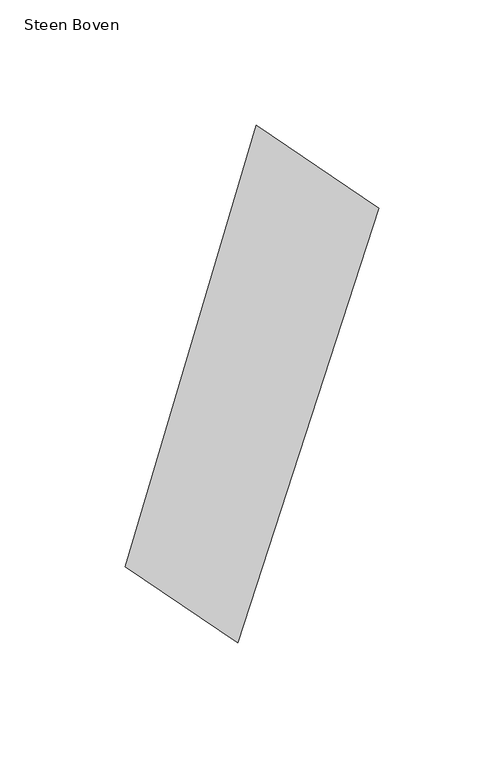
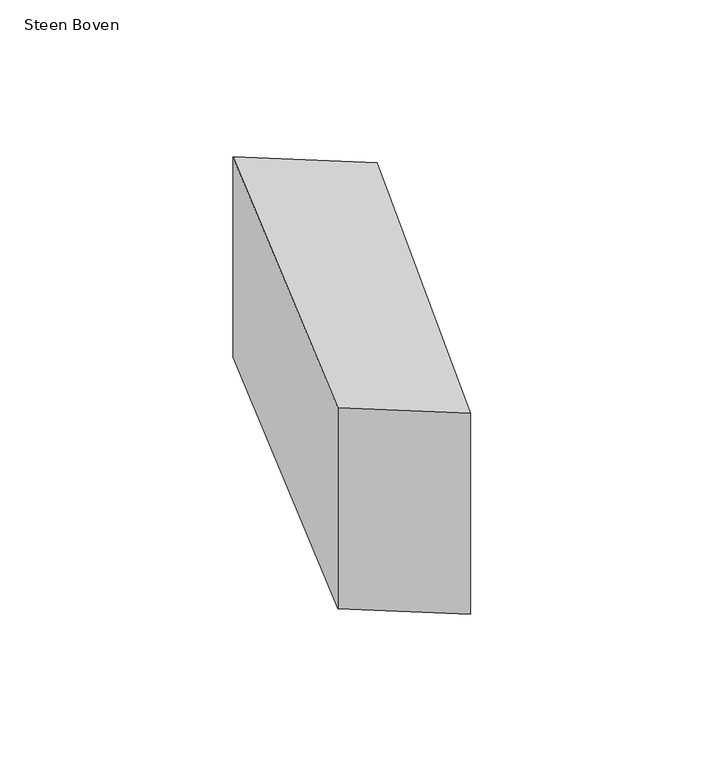
"""IFC4 building model written with IfcOpenShell, lengths in millimetres: proxy geometry, 00_GMA_steen_versie_4 : Steen Boven."""

import ifcopenshell
import ifcopenshell.guid

model = None  # the IFC model being written
_history = None  # IfcOwnerHistory: only IFC2X3 demands one
_inside = {}  # id of a spatial element -> (the spatial element, [elements in it])
_under = {}  # id of a project, library or spatial element -> (it, [spatial elements below it])
_declared = {}  # id of a project -> (the project, [libraries it declares])
_typed = {}  # id of a type object -> (the type object, [elements of that type])
_made_of = {}  # id of a material, layer set ... -> (it, [elements and type objects made of it])


def new_model(schema):
    """Start an empty IFC model of exactly this schema.

    Asked for "IFC4X3", IfcOpenShell would pick the latest addendum, in which some entities
    have other attributes; the version numbers below select the first issue.
    IFC2X3 requires an IfcOwnerHistory on every rooted entity: one is made here for all.
    """
    global model, _history
    if schema == "IFC4X3":
        model = ifcopenshell.file(schema_version=(4, 3, 0, 0))
    else:
        model = ifcopenshell.file(schema=schema)
    _inside.clear()
    _under.clear()
    _declared.clear()
    _typed.clear()
    _made_of.clear()
    _history = None
    if model.schema == "IFC2X3":
        org = make("IfcOrganization", Name="unknown")
        user = make(
            "IfcPersonAndOrganization",
            ThePerson=make("IfcPerson", FamilyName="unknown"),
            TheOrganization=org,
        )
        app = make(
            "IfcApplication",
            ApplicationDeveloper=org,
            Version="unknown",
            ApplicationFullName="unknown",
            ApplicationIdentifier="unknown",
        )
        _history = make(
            "IfcOwnerHistory",
            OwningUser=user,
            OwningApplication=app,
            ChangeAction="ADDED",
            CreationDate=0,
        )
    return model


def make(cls, **values):
    """One entity of the class cls with the attributes given. An attribute that is None is left unset."""
    return model.create_entity(
        cls, **{name: value for name, value in values.items() if value is not None}
    )


def rooted(cls, **values):
    """An entity with a GlobalId (a new one), such as an element, a storey or a relation."""
    return make(cls, GlobalId=ifcopenshell.guid.new(), OwnerHistory=_history, **values)


def si_unit(unit_type, name, prefix=None):
    """IfcSIUnit, for example si_unit("LENGTHUNIT", "METRE", prefix="MILLI")."""
    return make("IfcSIUnit", UnitType=unit_type, Prefix=prefix, Name=name)


def assignment(units):
    """IfcUnitAssignment: the units of a project."""
    return None if units is None else make("IfcUnitAssignment", Units=units)


def point(xyz):
    """IfcCartesianPoint."""
    return None if xyz is None else make("IfcCartesianPoint", Coordinates=xyz)


def direction(xyz):
    """IfcDirection."""
    return None if xyz is None else make("IfcDirection", DirectionRatios=xyz)


def frame(location, z_axis=None, x_axis=None):
    """IfcAxis2Placement3D, a coordinate frame: its origin and axes. An axis left out is left unset."""
    return make(
        "IfcAxis2Placement3D",
        Location=point(location),
        Axis=direction(z_axis),
        RefDirection=direction(x_axis),
    )


def origin():
    """The frame at (0, 0, 0) with its axes left unset."""
    return frame((0.0, 0.0, 0.0))


def origin_with_axes():
    """The frame at (0, 0, 0) with the z axis (0, 0, 1) and the x axis (1, 0, 0) written out."""
    return frame((0.0, 0.0, 0.0), z_axis=(0.0, 0.0, 1.0), x_axis=(1.0, 0.0, 0.0))


def place(relative_to, where):
    """IfcLocalPlacement: puts the frame where relative to a parent placement (None: the world)."""
    return make(
        "IfcLocalPlacement", PlacementRelTo=relative_to, RelativePlacement=where
    )


def context(
    kind, dimensions, precision=None, world=None, true_north=None, identifier=None
):
    """IfcGeometricRepresentationContext, for example the 3D "Model" context."""
    return make(
        "IfcGeometricRepresentationContext",
        ContextIdentifier=identifier,
        ContextType=kind,
        CoordinateSpaceDimension=dimensions,
        Precision=precision,
        WorldCoordinateSystem=world,
        TrueNorth=true_north,
    )


def project(units=None, contexts=None):
    """IfcProject with its units and contexts."""
    return rooted(
        "IfcProject",
        Name="project",
        RepresentationContexts=contexts,
        UnitsInContext=assignment(units),
    )


def spatial(cls, under=None, at=None, **own):
    """A site, building, storey or space (cls), placed at a placement, below another one or the project."""
    s = rooted(cls, ObjectPlacement=at, **own)
    if under is not None:
        _under.setdefault(under.id(), (under, []))[1].append(s)
    return s


def polyline(points):
    """IfcPolyline through the points."""
    return make("IfcPolyline", Points=[point(p) for p in points])


def outline(outer, holes=None, kind="AREA"):
    """IfcArbitraryClosedProfileDef: a profile drawn as a closed curve; with holes, ...WithVoids."""
    if holes is None:
        return make("IfcArbitraryClosedProfileDef", ProfileType=kind, OuterCurve=outer)
    return make(
        "IfcArbitraryProfileDefWithVoids",
        ProfileType=kind,
        OuterCurve=outer,
        InnerCurves=holes,
    )


def extrude(swept, where, along, depth):
    """IfcExtrudedAreaSolid: the profile swept, set in the frame where, extruded along a direction by depth."""
    return make(
        "IfcExtrudedAreaSolid",
        SweptArea=swept,
        Position=where,
        ExtrudedDirection=direction(along),
        Depth=depth,
    )


def shape(context_of_items, identifier, shape_type, items):
    """IfcShapeRepresentation: the items that make up one representation, for example the "Body"."""
    return make(
        "IfcShapeRepresentation",
        ContextOfItems=context_of_items,
        RepresentationIdentifier=identifier,
        RepresentationType=shape_type,
        Items=items,
    )


def source(mapping_origin, context_of_items, identifier, shape_type, items):
    """IfcRepresentationMap: a shape defined once, which mapped items show again and again."""
    return make(
        "IfcRepresentationMap",
        MappingOrigin=mapping_origin,
        MappedRepresentation=shape(context_of_items, identifier, shape_type, items),
    )


def transform(
    local_origin,
    x_axis=None,
    y_axis=None,
    z_axis=None,
    scale=None,
    scale2=None,
    scale3=None,
    uniform=True,
):
    """IfcCartesianTransformationOperator3D, or its non-uniform kind. x_axis, y_axis, z_axis: its Axis1, 2, 3."""
    if uniform:
        return make(
            "IfcCartesianTransformationOperator3D",
            Axis1=direction(x_axis),
            Axis2=direction(y_axis),
            LocalOrigin=point(local_origin),
            Scale=scale,
            Axis3=direction(z_axis),
        )
    return make(
        "IfcCartesianTransformationOperator3DnonUniform",
        Axis1=direction(x_axis),
        Axis2=direction(y_axis),
        LocalOrigin=point(local_origin),
        Scale=scale,
        Axis3=direction(z_axis),
        Scale2=scale2,
        Scale3=scale3,
    )


def mapped(mapping_source, mapping_target):
    """IfcMappedItem: shows the shape of a source again, moved by a transform."""
    return make(
        "IfcMappedItem", MappingSource=mapping_source, MappingTarget=mapping_target
    )


def made_of(thing, what):
    """Note that an element or type object is made of a material, layer set ...; save() writes the relation."""
    if what is not None:
        _made_of.setdefault(what.id(), (what, []))[1].append(thing)
    return thing


def element(
    cls,
    number,
    at=None,
    inside=None,
    cuts=None,
    type_object=None,
    material=None,
    context=None,
    identifier="Body",
    shape_type=None,
    held_by="IfcProductDefinitionShape",
    body=None,
    shapes=None,
    **own,
):
    """One element of the class cls, such as IfcWall. Its Tag is "e" and its number.

    at: its placement. inside: the storey or other place that contains it. cuts: it is an
    opening in that element (IfcRelVoidsElement). A single representation is given by context,
    identifier, shape_type and body (its items); several are given by shapes. held_by: the class
    of the entity that holds the representations. save() writes the other relations.
    """
    e = rooted(cls, Tag="e%d" % number, ObjectPlacement=at, **own)
    if body is not None:
        shapes = [shape(context, identifier, shape_type, body)]
    if shapes is not None:
        e.Representation = make(held_by, Representations=shapes)
    if inside is not None:
        _inside.setdefault(inside.id(), (inside, []))[1].append(e)
    if cuts is not None:
        rooted(
            "IfcRelVoidsElement", RelatingBuildingElement=cuts, RelatedOpeningElement=e
        )
    if type_object is not None:
        _typed.setdefault(type_object.id(), (type_object, []))[1].append(e)
    return made_of(e, material)


def aggregate(whole, parts):
    """IfcRelAggregates: a whole, such as a stair, and the parts it consists of."""
    return rooted("IfcRelAggregates", RelatingObject=whole, RelatedObjects=parts)


def save(model, path):
    """Write the relations noted so far, then the file.

    IfcRelAggregates (storeys below a building ...), IfcRelContainedInSpatialStructure (elements
    in a storey), IfcRelDefinesByType, IfcRelAssociatesMaterial and IfcRelDeclares: one each for
    every whole, place, type object, material and project.
    """
    for whole, parts in _under.values():
        aggregate(whole, parts)
    for where, things in _inside.values():
        rooted(
            "IfcRelContainedInSpatialStructure",
            RelatedElements=things,
            RelatingStructure=where,
        )
    for kind, things in _typed.values():
        rooted("IfcRelDefinesByType", RelatedObjects=things, RelatingType=kind)
    for what, things in _made_of.values():
        rooted("IfcRelAssociatesMaterial", RelatedObjects=things, RelatingMaterial=what)
    for by, libraries in _declared.values():
        rooted("IfcRelDeclares", RelatingContext=by, RelatedDefinitions=libraries)
    model.write(path)


def steen_boven_d78be7b2(model_context):
    return source(origin(), model_context, "Body", "SweptSolid", [
        extrude(outline(polyline([(130.3284375, 160.5281469), (74.0412724, -12.9715113), (29.2233588, 17.3669544), (81.5175375, 193.610291), (130.3284375, 160.5281469)])), origin_with_axes(), (0.0, 0.0, 1.0), 100.0),
    ])


if __name__ == "__main__":
    model = new_model("IFC4")
    model_context = context("Model", 3, world=origin())
    ifc_project = project(units=[si_unit("LENGTHUNIT", "METRE", prefix="MILLI")], contexts=[model_context])
    site = spatial("IfcSite", under=ifc_project)
    building = spatial("IfcBuilding", under=site)
    placement = place(None, origin())
    steen_boven_shape = steen_boven_d78be7b2(model_context)
    element("IfcBuildingElementProxy", 1, Name="00_GMA_steen_versie_4 : Steen Boven", ObjectType="00_GMA_steen_versie_4 : Steen Boven", at=placement, inside=building, context=model_context, shape_type="MappedRepresentation", body=[
        mapped(steen_boven_shape, transform((0.0, 0.0, 0.0), x_axis=(1.0, 0.0, 0.0), y_axis=(0.0, 1.0, 0.0), z_axis=(0.0, 0.0, 1.0))),
    ])
    save(model, "model.ifc")

# Revit data of these elements
# Type "00_GMA_steen_versie_4 : Steen Boven"
#   StootVoegHalfBoven [instance default] = 5 mm
#   StootVoegHalf [instance default] = 5 mm
#   StootVoegBreedteOnder = 10 mm
#   StootVoegBreedteBoven = 10 mm
#   Steendikte = 100 mm
#   LintVoegOnderHalf = 5 mm
#   LintVoegOnder = 10 mm
#   LintVoegBovenHalf = 0 mm
#   LintVoegBoven = 0 mm
#   materiaal = none
#   MateriaalVoeg = none
#   Default Elevation = 0
